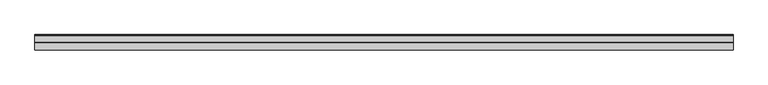
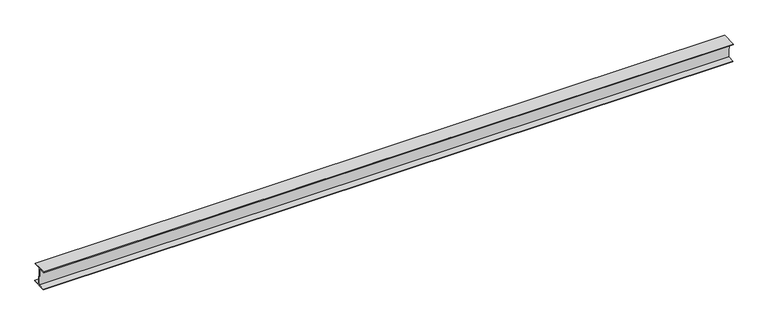
"""IFC4 building model written with IfcOpenShell, lengths in millimetres: proxy geometry, Generic Models 7:Generic Models 1:8:Generic Models 1:8 : Generic Models 7:Generic Models 1:337419:12 : Generic Models 7:Generic Models 1:8:Generic Models 1:8 : Generic Models 7:Generic Models 1:337419:315935."""

from ifc_helpers import new_model, si_unit, frame, origin, place, context, project, spatial, polyline, outline, extrude, source, transform, mapped, element, save


def generic_models_469aba90(model_context):
    return source(origin(), model_context, "Body", "SweptSolid", [
        extrude(outline(polyline([(-575826.8297655, 4049.9332877), (-575827.1021742, 4056.7858753), (-575674.8224487, 4062.8394016), (-575674.55004, 4055.986814), (-575747.771208, 4053.0760768), (-575740.244657, 3863.741618), (-575667.0419524, 3866.6516212), (-575666.7695437, 3859.7990336), (-575819.0492693, 3853.7455073), (-575819.3216779, 3860.5980949), (-575746.335846, 3863.4994769), (-575753.862397, 4052.8339357), (-575826.8297655, 4049.9332877)])), frame((588867.6367239, 0.0, 0.0), z_axis=(1.0, 0.0, 0.0), x_axis=(0.0, 1.0, 0.0)), (0.0, 0.0, 1.0), 7315.2),
    ])


if __name__ == "__main__":
    model = new_model("IFC4")
    model_context = context("Model", 3, world=origin())
    ifc_project = project(units=[si_unit("LENGTHUNIT", "METRE", prefix="MILLI")], contexts=[model_context])
    site = spatial("IfcSite", under=ifc_project)
    building = spatial("IfcBuilding", under=site)
    placement = place(None, origin())
    generic_models_shape = generic_models_469aba90(model_context)
    element("IfcBuildingElementProxy", 1, Name="Generic Models 7:Generic Models 1:8:Generic Models 1:8 : Generic Models 7:Generic Models 1:337419:12 : Generic Models 7:Generic Models 1:8:Generic Models 1:8 : Generic Models 7:Generic Models 1:337419:315935", ObjectType="Generic Models 7:Generic Models 1:8:Generic Models 1:8 : Generic Models 7:Generic Models 1:337419:12 : Generic Models 7:Generic Models 1:8:Generic Models 1:8 : Generic Models 7:Generic Models 1:337419:315935", at=placement, inside=building, context=model_context, shape_type="MappedRepresentation", body=[
        mapped(generic_models_shape, transform((0.0, 0.0, 0.0), x_axis=(1.0, 0.0, 0.0), y_axis=(0.0, 1.0, 0.0), z_axis=(0.0, 0.0, 1.0))),
    ])
    save(model, "model.ifc")

# Revit data of these elements
# Type "Generic Models 7:Generic Models 1:8:Generic Models 1:8 : Generic Models 7:Generic Models 1:337419:12 : Generic Models 7:Generic Models 1:8:Generic Models 1:8 : Generic Models 7:Generic Models 1:337419:315935"
#   NameOverride = "Generic Models 7:Generic Models 1:8:Generic Models 1:8 : Generic Models 7:Generic Models 1:337419:315935"
#   ObjectTypeOverride = "Generic Models 1:8 : Generic Models 7:Generic Models 1:337419"
#   Reference = "Generic Models 1"
#   Tag = "315935"
# Element 1 (IfcBuildingElementProxy, "Generic Models 7:Generic Models 1:8:Generic Models 1:8 : Generic Models 7:Generic Models 1:337419:12 : Generic Models 7:Generic Models 1:8:Generic Models 1:8 : Generic Models 7:Generic Models 1:337419:315935")
#   Materials on its faces: "STRUCTURAL STEEL - SEE STRUCT. DWGS"
# Materials
#   "STRUCTURAL STEEL - SEE STRUCT. DWGS": class "Metal", colour RGB 189 187 185, transparency 0, Description = "Structural steel 50ksi", Cost = 0
